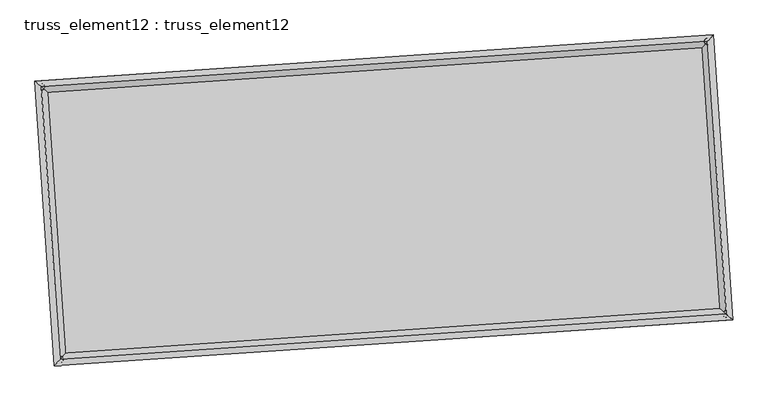
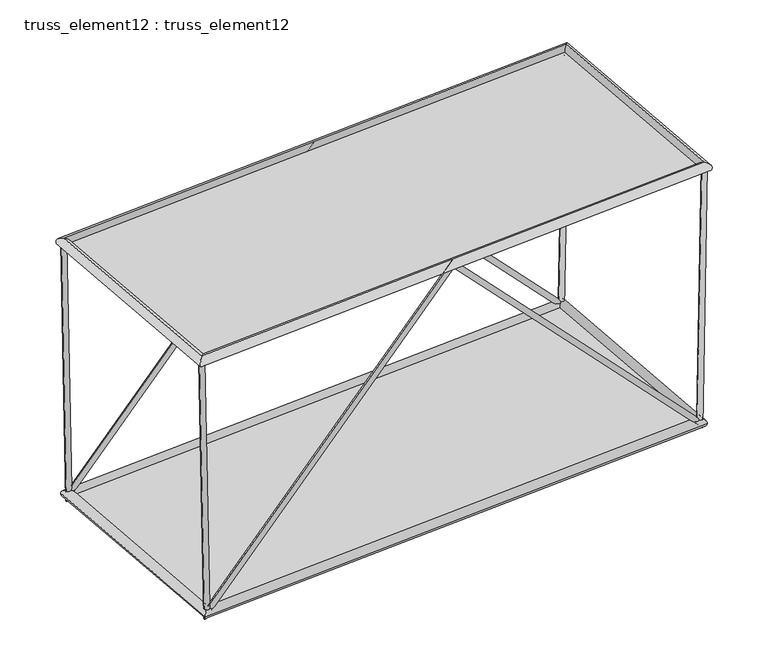
"""IFC4 building model written with IfcOpenShell, lengths in millimetres: plate geometry, truss_element12 : truss_element12."""

from ifc_helpers import new_model, si_unit, frame, origin, origin_with_axes, place, context, project, spatial, polyline, circle_curve, ellipse_curve, outline, extrude, source, transform, mapped, element, save
from ifc_brep_helpers import plane_surface, cylinder_surface, advanced_brep


def truss_element12_truss_element12_4f4fbcf4(model_context):
    return source(origin(), model_context, "Body", "SolidModel", [
        advanced_brep(
        [(-3760.412313, 2269.7141982, 5000.0391427), (-3859.4974462, 2256.3541767, 4998.1296386), (-3667.2581462, 2276.0660267, 121.7809681), (-3761.7287366, 2263.0206534, -121.7809681), (1063.0131777, 2598.6052469, 5071.2149086), (1063.4719257, 2592.0327442, 4926.9805708), (5794.6632736, 2921.2384802, 121.7906375), (5890.0977034, 2921.1420083, -121.7906375), (5886.4489476, 2927.4969964, 5000.0518193), (5986.4310183, 2927.7106108, 4998.1703582)],
        [
            (0, 1, circle_curve(frame((-3809.9548796, 2263.0341875, 4999.0843906), z_axis=(-0.01909228763423125, -0.001301830517198407, 0.9998168781282883), x_axis=(-0.13360060813890293, 0.9910344534146752, -0.0012608132261237302)), 50.0)),
            (1, 0, circle_curve(frame((-3809.9548796, 2263.0341875, 4999.0843906), z_axis=(-0.01909228763423125, -0.001301830517198407, 0.9998168781282883), x_axis=(-0.13360060813890293, 0.9910344534146752, -0.0012608132261237302)), 50.0)),
            (0, 2),
            (2, 3, ellipse_curve(frame((-3714.4934414, 2269.54334, 0.0), z_axis=(-0.9293023610631932, -0.06336559539190412, 0.36384326713985493), x_axis=(0.36300038639906895, 0.02475161645489898, 0.9314601853847518)), 131.026691, 50.0)),
            (3, 1),
            (3, 2, ellipse_curve(frame((-3714.4934414, 2269.54334, 0.0), z_axis=(-0.9293023610631932, -0.06336559539190412, 0.36384326713985493), x_axis=(0.36300038639906895, 0.02475161645489898, 0.9314601853847518)), 131.026691, 50.0)),
            (2, 4),
            (4, 5, ellipse_curve(frame((1063.2425517, 2595.3189955, 4999.0977397), z_axis=(-0.9976833933961032, -0.0680282380460461, -7.328019523158009e-05), x_axis=(7.311043404377707e-05, 4.985122578964847e-06, -0.9999999973150066)), 72.2742041, 50.0)),
            (5, 3),
            (5, 4, ellipse_curve(frame((1063.2425517, 2595.3189955, 4999.0977397), z_axis=(-0.9976833933961032, -0.0680282380460461, -7.328019523158009e-05), x_axis=(7.311043404377707e-05, 4.985122578964847e-06, -0.9999999973150066)), 72.2742041, 50.0)),
            (4, 6),
            (6, 7, ellipse_curve(frame((5842.3804885, 2921.1902443, 0.0), z_axis=(-0.9292247210951414, -0.06336030141762011, -0.36404242872215437), x_axis=(-0.36319908660286526, -0.02476516506646599, 0.9313823651380109)), 131.0480431, 50.0)),
            (7, 5),
            (7, 6, ellipse_curve(frame((5842.3804885, 2921.1902443, 0.0), z_axis=(-0.9292247210951414, -0.06336030141762011, -0.36404242872215437), x_axis=(-0.36319908660286526, -0.02476516506646599, 0.9313823651380109)), 131.0480431, 50.0)),
            (8, 9, circle_curve(frame((5936.4399829, 2927.6038036, 4999.1110888), z_axis=(0.018811898886609116, 0.0012827118743552863, 0.9998222177519999), x_axis=(-0.002159898325700627, 0.9999968957639224, -0.001242296961952952)), 50.0)),
            (9, 8, circle_curve(frame((5936.4399829, 2927.6038036, 4999.1110888), z_axis=(0.018811898886609116, 0.0012827118743552863, 0.9998222177519999), x_axis=(-0.002159898325700627, 0.9999968957639224, -0.001242296961952952)), 50.0)),
            (6, 8),
            (9, 7),
        ],
        [
            plane_surface(frame((-3809.9548796, 2313.0341451, 4999.149494), z_axis=(-0.019092287634232964, -0.0013018305172036876, 0.9998168781282883), x_axis=(0.9998177256644792, -2.4859453925607497e-05, 0.01909227144987823))),
            cylinder_surface(frame((-3809.9548796, 2263.0341875, 4999.0843906), z_axis=(-0.019092287634231247, -0.0013018305171984068, 0.9998168781282881), x_axis=(-0.13360060813890293, 0.9910344534146752, -0.0012608132261237302)), 50.0),
            cylinder_surface(frame((-3714.4934414, 2269.54334, 0.0), z_axis=(-0.690154320065974, -0.047058999563115655, -0.7221305041710897), x_axis=(-0.020413190140967315, 0.9987522731822975, -0.04557629297630685)), 50.0),
            cylinder_surface(frame((1063.2425517, 2595.3189955, 4999.0977397), z_axis=(-0.6902599032026433, -0.04706619887584647, 0.7220291122621422), x_axis=(-0.11534100259403575, 0.9922795065055209, -0.04558326545743215)), 50.0),
            plane_surface(frame((5936.4399829, 2877.6038448, 4999.1752357), z_axis=(0.018811898886608048, 0.0012827118743585436, 0.9998222177519999), x_axis=(0.9998230405728206, -2.41345169111895e-05, -0.018811883405046356))),
            cylinder_surface(frame((5842.3804885, 2921.1902443, 0.0), z_axis=(-0.018811898886609116, -0.0012827118743552863, -0.9998222177519999), x_axis=(-0.002159898325700627, 0.9999968957639224, -0.001242296961952952)), 50.0),
        ],
        [
            (0, [[1, 2]]),
            (1, [[-1, 3, 4, 5]]),
            (1, [[-2, -5, 6, -3]]),
            (2, [[-4, 7, 8, 9]]),
            (2, [[-6, -9, 10, -7]]),
            (3, [[-8, 11, 12, 13]]),
            (3, [[-10, -13, 14, -11]]),
            (4, [[15, 16]]),
            (5, [[-12, 17, -16, 18]]),
            (5, [[-14, -18, -15, -17]]),
        ],
    ),
        advanced_brep(
        [(-3488.2993601, -1721.0193861, 5000.0391427), (-3587.3844933, -1734.3794076, 4998.1296386), (-3395.1451933, -1714.6675576, 121.7809681), (-3489.6157837, -1727.7129309, -121.7809681), (1335.1261306, -1392.1283374, 5071.2149086), (1335.5848786, -1398.7008401, 4926.9805708), (6066.7762265, -1069.4951041, 121.7906375), (6162.2106563, -1069.591576, -121.7906375), (6158.5619005, -1063.2365879, 5000.0518193), (6258.5439712, -1063.0229735, 4998.1703582)],
        [
            (0, 1, circle_curve(frame((-3537.8419267, -1727.6993968, 4999.0843906), z_axis=(-0.019092287634231597, -0.0013018305171984207, 0.9998168781282882), x_axis=(-0.13360060813890337, 0.9910344534146753, -0.001260813226123772)), 50.0)),
            (1, 0, circle_curve(frame((-3537.8419267, -1727.6993968, 4999.0843906), z_axis=(-0.019092287634231597, -0.0013018305171984207, 0.9998168781282882), x_axis=(-0.13360060813890337, 0.9910344534146753, -0.001260813226123772)), 50.0)),
            (0, 2),
            (2, 3, ellipse_curve(frame((-3442.3804885, -1721.1902443, 0.0), z_axis=(-0.9293023610631933, -0.06336559539190433, 0.36384326713985427), x_axis=(0.3630003863990683, 0.02475161645489903, 0.9314601853847522)), 131.026691, 50.0)),
            (3, 1),
            (3, 2, ellipse_curve(frame((-3442.3804885, -1721.1902443, 0.0), z_axis=(-0.9293023610631933, -0.06336559539190433, 0.36384326713985427), x_axis=(0.3630003863990683, 0.02475161645489903, 0.9314601853847522)), 131.026691, 50.0)),
            (2, 4),
            (4, 5, ellipse_curve(frame((1335.3555046, -1395.4145888, 4999.0977397), z_axis=(-0.9976833933961031, -0.06802823804604609, -7.328019523141967e-05), x_axis=(7.311043404362326e-05, 4.985122578705385e-06, -0.9999999973150066)), 72.2742041, 50.0)),
            (5, 3),
            (5, 4, ellipse_curve(frame((1335.3555046, -1395.4145888, 4999.0977397), z_axis=(-0.9976833933961031, -0.06802823804604609, -7.328019523141967e-05), x_axis=(7.311043404362326e-05, 4.985122578705385e-06, -0.9999999973150066)), 72.2742041, 50.0)),
            (4, 6),
            (6, 7, ellipse_curve(frame((6114.4934414, -1069.54334, 0.0), z_axis=(-0.9292247210951415, -0.06336030141762007, -0.36404242872215387), x_axis=(-0.3631990866028648, -0.024765165066465773, 0.9313823651380111)), 131.0480431, 50.0)),
            (7, 5),
            (7, 6, ellipse_curve(frame((6114.4934414, -1069.54334, 0.0), z_axis=(-0.9292247210951415, -0.06336030141762007, -0.36404242872215387), x_axis=(-0.3631990866028648, -0.024765165066465773, 0.9313823651380111)), 131.0480431, 50.0)),
            (8, 9, circle_curve(frame((6208.5529358, -1063.1297807, 4999.1110888), z_axis=(0.018811898886609498, 0.0012827118743554589, 0.9998222177519999), x_axis=(-0.002159898325700537, 0.9999968957639224, -0.0012422969619531254)), 50.0)),
            (9, 8, circle_curve(frame((6208.5529358, -1063.1297807, 4999.1110888), z_axis=(0.018811898886609498, 0.0012827118743554589, 0.9998222177519999), x_axis=(-0.002159898325700537, 0.9999968957639224, -0.0012422969619531254)), 50.0)),
            (6, 8),
            (9, 7),
        ],
        [
            plane_surface(frame((-3537.8419267, -1677.6994392, 4999.149494), z_axis=(-0.019092287634232964, -0.001301830517203691, 0.9998168781282883), x_axis=(0.9998177256644792, -2.4859453925607497e-05, 0.01909227144987823))),
            cylinder_surface(frame((-3537.8419267, -1727.6993968, 4999.0843906), z_axis=(-0.0190922876342316, -0.001301830517198421, 0.9998168781282885), x_axis=(-0.13360060813890337, 0.9910344534146753, -0.001260813226123772)), 50.0),
            cylinder_surface(frame((-3442.3804885, -1721.1902443, 0.0), z_axis=(-0.6901543200659737, -0.047058999563115794, -0.7221305041710899), x_axis=(-0.02041319014096742, 0.9987522731822974, -0.04557629297630694)), 50.0),
            cylinder_surface(frame((1335.3555046, -1395.4145888, 4999.0977397), z_axis=(-0.6902599032026426, -0.04706619887584624, 0.7220291122621428), x_axis=(-0.11534100259403567, 0.9922795065055209, -0.045583265457432236)), 50.0),
            plane_surface(frame((6208.5529358, -1113.1297395, 4999.1752357), z_axis=(0.018811898886608048, 0.0012827118743585436, 0.9998222177519999), x_axis=(0.9998230405728206, -2.41345169111895e-05, -0.018811883405046356))),
            cylinder_surface(frame((6114.4934414, -1069.54334, 0.0), z_axis=(-0.018811898886609498, -0.0012827118743554589, -0.9998222177519999), x_axis=(-0.002159898325700537, 0.9999968957639224, -0.0012422969619531254)), 50.0),
        ],
        [
            (0, [[1, 2]]),
            (1, [[-1, 3, 4, 5]]),
            (1, [[-2, -5, 6, -3]]),
            (2, [[-4, 7, 8, 9]]),
            (2, [[-6, -9, 10, -7]]),
            (3, [[-8, 11, 12, 13]]),
            (3, [[-10, -13, 14, -11]]),
            (4, [[15, 16]]),
            (5, [[-12, 17, -16, 18]]),
            (5, [[-14, -18, -15, -17]]),
        ],
    ),
        advanced_brep(
        [(-3537.8349665, -1727.6916826, 4909.084391), (-3537.8488868, -1727.7071111, 5089.0843903), (-3809.9628225, 2263.0408855, 5089.0843903), (-3809.9469367, 2263.0274894, 4909.084391), (5936.4464523, 2927.6114844, 5089.1110885), (5936.4335136, 2927.5961229, 4909.111089), (6208.5603879, -1063.1365122, 5089.1110885), (6208.5454838, -1063.1230492, 4909.111089)],
        [
            (0, 1, ellipse_curve(frame((-3537.8419267, -1727.6993968, 4999.0843906), z_axis=(-0.7535719234028239, 0.6573654662782598, -1.9324773013398396e-06), x_axis=(-0.6573654662754455, -0.753571923405279, -1.9324773013398426e-06)), 127.2792206, 90.0)),
            (1, 2),
            (2, 3, ellipse_curve(frame((-3809.9548796, 2263.0341875, 4999.0843906), z_axis=(-0.6573654662754456, -0.753571923405279, -1.9324773013398405e-06), x_axis=(0.753571923402824, -0.6573654662782596, 1.932477301339838e-06)), 127.2792206, 90.0)),
            (3, 0),
            (1, 0, ellipse_curve(frame((-3537.8419267, -1727.6993968, 4999.0843906), z_axis=(-0.7535719234028239, 0.6573654662782598, -1.9324773013398396e-06), x_axis=(-0.6573654662754455, -0.753571923405279, -1.9324773013398426e-06)), 127.2792206, 90.0)),
            (3, 2, ellipse_curve(frame((-3809.9548796, 2263.0341875, 4999.0843906), z_axis=(-0.6573654662754456, -0.753571923405279, -1.9324773013398405e-06), x_axis=(0.753571923402824, -0.6573654662782596, 1.932477301339838e-06)), 127.2792206, 90.0)),
            (2, 4),
            (4, 5, ellipse_curve(frame((5936.4399829, 2927.6038036, 4999.1110888), z_axis=(-0.7535719234028233, 0.6573654662782605, -1.9324773013398405e-06), x_axis=(-0.6573654662754463, -0.753571923405278, -1.9324773013398375e-06)), 127.2792206, 90.0)),
            (5, 3),
            (5, 4, ellipse_curve(frame((5936.4399829, 2927.6038036, 4999.1110888), z_axis=(-0.7535719234028233, 0.6573654662782605, -1.9324773013398405e-06), x_axis=(-0.6573654662754463, -0.753571923405278, -1.9324773013398375e-06)), 127.2792206, 90.0)),
            (4, 6),
            (6, 7, ellipse_curve(frame((6208.5529358, -1063.1297807, 4999.1110888), z_axis=(0.6573654662754466, 0.753571923405278, 1.9324773013398396e-06), x_axis=(-0.7535719234028231, 0.6573654662782609, -1.9324773013398426e-06)), 127.2792206, 90.0)),
            (7, 5),
            (7, 6, ellipse_curve(frame((6208.5529358, -1063.1297807, 4999.1110888), z_axis=(0.6573654662754466, 0.753571923405278, 1.9324773013398396e-06), x_axis=(-0.7535719234028231, 0.6573654662782609, -1.9324773013398426e-06)), 127.2792206, 90.0)),
            (6, 1),
            (0, 7),
        ],
        [
            cylinder_surface(frame((-3537.8419267, -1727.6993968, 4999.0843906), z_axis=(0.06802823822870284, -0.9976833960748765, 0.0), x_axis=(-0.9976833926394355, -0.06802823799445316, -8.298696276640426e-05)), 90.0),
            cylinder_surface(frame((-3809.9548796, 2263.0341875, 4999.0843906), z_axis=(-0.9976833960711509, -0.06802823822844752, -2.732935608532959e-06), x_axis=(-0.06802823779080554, 0.997683392876903, -8.025402716667233e-05)), 90.0),
            cylinder_surface(frame((5936.4399829, 2927.6038036, 4999.1110888), z_axis=(-0.06802823822870042, 0.9976833960748767, 0.0), x_axis=(0.9976833930770777, 0.0680282380242919, -7.752109156694041e-05)), 90.0),
            cylinder_surface(frame((6208.5529358, -1063.1297807, 4999.1110888), z_axis=(0.9976833960711509, 0.0680282382284473, 2.732935608532962e-06), x_axis=(0.0680282382284473, -0.997683392847062, -8.025402716667235e-05)), 90.0),
        ],
        [
            (0, [[1, 2, 3, 4]]),
            (0, [[5, -4, 6, -2]]),
            (1, [[-3, 7, 8, 9]]),
            (1, [[-6, -9, 10, -7]]),
            (2, [[-8, 11, 12, 13]]),
            (2, [[-10, -13, 14, -11]]),
            (3, [[-12, 15, -1, 16]]),
            (3, [[-14, -16, -5, -15]]),
        ],
    ),
        advanced_brep(
        [(-3358.7115243, -1625.2761972, 0.0), (-3526.0494527, -1817.1042913, 0.0), (-3810.4074885, 2353.2123043, 0.0), (-3618.5793943, 2185.8743758, 0.0), (5926.0494527, 3017.1042913, 0.0), (5758.7115243, 2825.2761972, 0.0), (6210.4074885, -1153.2123043, 0.0), (6018.5793943, -985.8743758, 0.0)],
        [
            (0, 1, ellipse_curve(frame((-3442.3804885, -1721.1902443, 0.0), z_axis=(-0.7535719234054584, 0.6573654662780802, 0.0), x_axis=(-0.6573654662780803, -0.7535719234054584, 0.0)), 127.2792206, 90.0)),
            (1, 2),
            (2, 3, ellipse_curve(frame((-3714.4934414, 2269.54334, 0.0), z_axis=(-0.65736546627808, -0.7535719234054585, 0.0), x_axis=(0.7535719234054585, -0.6573654662780801, 0.0)), 127.2792206, 90.0)),
            (3, 0),
            (1, 0, ellipse_curve(frame((-3442.3804885, -1721.1902443, 0.0), z_axis=(-0.7535719234054584, 0.6573654662780802, 0.0), x_axis=(-0.6573654662780803, -0.7535719234054584, 0.0)), 127.2792206, 90.0)),
            (3, 2, ellipse_curve(frame((-3714.4934414, 2269.54334, 0.0), z_axis=(-0.65736546627808, -0.7535719234054585, 0.0), x_axis=(0.7535719234054585, -0.6573654662780801, 0.0)), 127.2792206, 90.0)),
            (2, 4),
            (4, 5, ellipse_curve(frame((5842.3804885, 2921.1902443, 0.0), z_axis=(-0.7535719234054579, 0.657365466278081, 0.0), x_axis=(-0.657365466278081, -0.7535719234054579, 0.0)), 127.2792206, 90.0)),
            (5, 3),
            (5, 4, ellipse_curve(frame((5842.3804885, 2921.1902443, 0.0), z_axis=(-0.7535719234054579, 0.657365466278081, 0.0), x_axis=(-0.657365466278081, -0.7535719234054579, 0.0)), 127.2792206, 90.0)),
            (4, 6),
            (6, 7, ellipse_curve(frame((6114.4934414, -1069.54334, 0.0), z_axis=(0.6573654662780812, 0.7535719234054576, 0.0), x_axis=(-0.7535719234054576, 0.6573654662780812, 0.0)), 127.2792206, 90.0)),
            (7, 5),
            (7, 6, ellipse_curve(frame((6114.4934414, -1069.54334, 0.0), z_axis=(0.6573654662780812, 0.7535719234054576, 0.0), x_axis=(-0.7535719234054576, 0.6573654662780812, 0.0)), 127.2792206, 90.0)),
            (6, 1),
            (0, 7),
        ],
        [
            cylinder_surface(frame((-3442.3804885, -1721.1902443, 0.0), z_axis=(0.06802823822870306, -0.9976833960748764, 0.0), x_axis=(-0.9976833960748764, -0.06802823822870306, 0.0)), 90.0),
            cylinder_surface(frame((-3714.4934414, 2269.54334, 0.0), z_axis=(-0.9976833960748767, -0.06802823822870151, 0.0), x_axis=(-0.06802823822870151, 0.9976833960748767, 0.0)), 90.0),
            cylinder_surface(frame((5842.3804885, 2921.1902443, 0.0), z_axis=(-0.06802823822870056, 0.9976833960748768, 0.0), x_axis=(0.9976833960748768, 0.06802823822870056, 0.0)), 90.0),
            cylinder_surface(frame((6114.4934414, -1069.54334, 0.0), z_axis=(0.9976833960748768, 0.0680282382287009, 0.0), x_axis=(0.0680282382287009, -0.9976833960748768, 0.0)), 90.0),
        ],
        [
            (0, [[1, 2, 3, 4]]),
            (0, [[5, -4, 6, -2]]),
            (1, [[-3, 7, 8, 9]]),
            (1, [[-6, -9, 10, -7]]),
            (2, [[-8, 11, 12, 13]]),
            (2, [[-10, -13, 14, -11]]),
            (3, [[-12, 15, -1, 16]]),
            (3, [[-14, -16, -5, -15]]),
        ],
    ),
        extrude(outline(polyline([(-3442.3804885, -1721.1902443), (-3714.4934414, 2269.54334), (5842.3804885, 2921.1902443), (6114.4934414, -1069.54334), (-3442.3804885, -1721.1902443)])), origin_with_axes(), (0.0, 0.0, 1.0), 20.0),
        extrude(outline(polyline([(-2000.0, 4884.5129131), (2000.0, 4884.512913), (2000.0, -4884.5129131), (-2000.0, -4884.512913), (-2000.0, 4884.5129131)])), frame((1199.2990281, 599.9522034, 4999.0977397), z_axis=(-2.726604479175121e-06, -1.8591679464098493e-07, 0.9999999999962655), x_axis=(-0.0680282382287028, 0.9976833960748764, 0.0)), (0.0, 0.0, 1.0), 20.0),
    ])


if __name__ == "__main__":
    model = new_model("IFC4")
    model_context = context("Model", 3, world=origin())
    ifc_project = project(units=[si_unit("LENGTHUNIT", "METRE", prefix="MILLI")], contexts=[model_context])
    site = spatial("IfcSite", under=ifc_project)
    building = spatial("IfcBuilding", under=site)
    placement = place(None, origin())
    truss_element12_truss_element12_shape = truss_element12_truss_element12_4f4fbcf4(model_context)
    element("IfcPlate", 1, ObjectType="truss_element12 : truss_element12", at=placement, inside=building, context=model_context, shape_type="MappedRepresentation", body=[
        mapped(truss_element12_truss_element12_shape, transform((0.0, 0.0, 0.0), x_axis=(1.0, 0.0, 0.0), y_axis=(0.0, 1.0, 0.0), z_axis=(0.0, 0.0, 1.0))),
    ])
    save(model, "model.ifc")

# Revit data of these elements
# Type "truss_element12 : truss_element12"
#   steellbar1 = 90 mm
#   steelbar2 = 50 mm
#   offset1 = 5000 mm
#   M = Default Roof
# Element 1 (IfcPlate, "truss_element12 : truss_element12")
#   Materials on its faces: "Default Roof"
# Materials
#   "Default Roof": class "Miscellaneous", colour RGB 0 127 0, transparency 0, Comments = "Rendering appearance not upgraded Rendering appearance not upgraded ", Cost = 0
